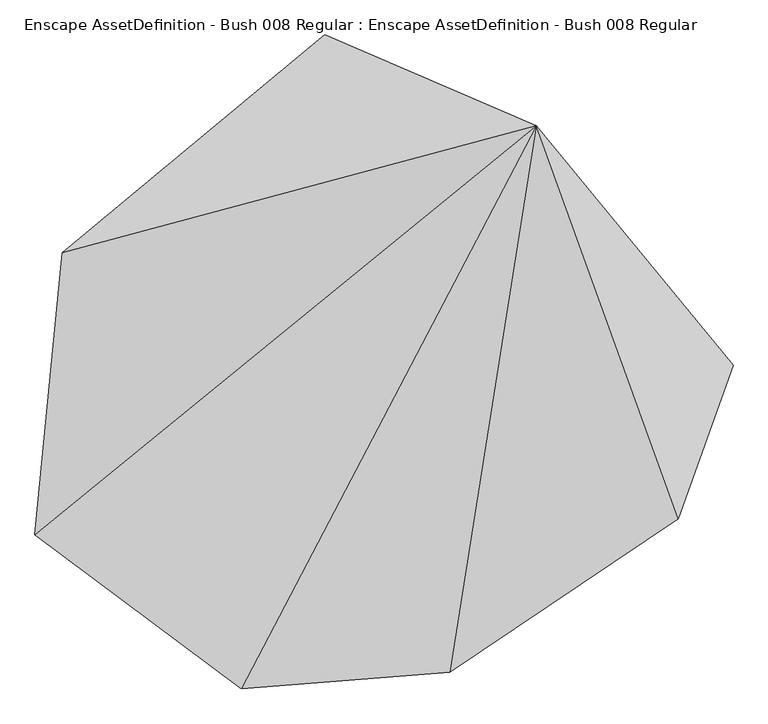
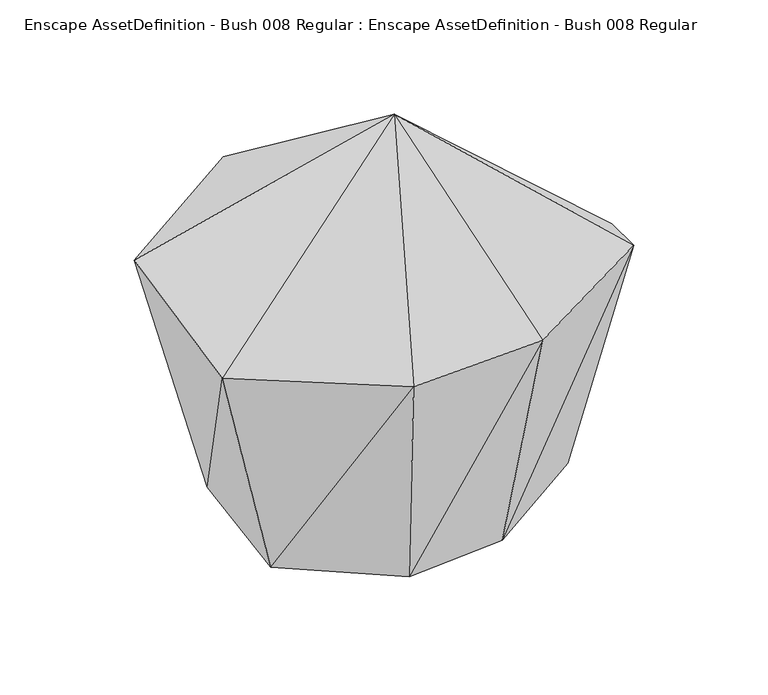
"""IFC4 building model written with IfcOpenShell, lengths in millimetres: geographic element geometry, Enscape AssetDefinition - Bush 008 Regular : Enscape AssetDefinition - Bush 008 Regular."""

from ifc_helpers import new_model, si_unit, origin, place, context, project, spatial, faceted_brep, source, transform, mapped, element, save


def enscape_assetdefinition_bush_008_regular_enscape_4d63b102(model_context):
    return source(origin(), model_context, "Body", "Brep", [
        faceted_brep([(-732.7302098, -362.3848855, 766.569972), (-488.0544245, 143.9245045, 0.0), (-529.4855833, -283.1877768, 0.0), (-675.306201, 229.6019644, 791.0672426), (-90.5457214, 473.4426737, 0.0), (229.8599929, 336.0404968, 0.0), (-300.0746369, -686.321795, 781.7997932), (-217.3293233, -516.9049501, 0.0), (319.7386861, 495.8788455, 779.6196342), (-124.3504807, 686.321795, 674.3021011), (527.8295279, -26.7513935, 0.0), (732.7302098, -6.9583626, 565.536499), (617.8262234, -329.4171691, 728.3439636), (138.3782178, -650.9299278, 766.2059665), (99.0101621, -491.3705885, 0.0), (444.9271858, -259.40153, 0.0)], [[[0, 1, 2]], [[3, 4, 1]], [[4, 5, 1]], [[1, 0, 3]], [[1, 5, 2]], [[6, 2, 7]], [[2, 6, 0]], [[2, 5, 7]], [[0, 8, 3]], [[8, 0, 6]], [[3, 8, 9]], [[4, 3, 9]], [[9, 5, 4]], [[5, 9, 8]], [[8, 10, 5]], [[11, 8, 12]], [[13, 8, 6]], [[8, 13, 12]], [[10, 8, 11]], [[7, 13, 6]], [[13, 7, 14]], [[7, 5, 14]], [[14, 12, 13]], [[12, 14, 15]], [[15, 11, 12]], [[11, 15, 10]], [[15, 5, 10]], [[14, 5, 15]]]),
    ])


if __name__ == "__main__":
    model = new_model("IFC4")
    model_context = context("Model", 3, world=origin())
    ifc_project = project(units=[si_unit("LENGTHUNIT", "METRE", prefix="MILLI")], contexts=[model_context])
    site = spatial("IfcSite", under=ifc_project)
    building = spatial("IfcBuilding", under=site)
    placement = place(None, origin())
    enscape_assetdefinition_bush_008_regular_enscape_shape = enscape_assetdefinition_bush_008_regular_enscape_4d63b102(model_context)
    element("IfcGeographicElement", 1, ObjectType="Enscape AssetDefinition - Bush 008 Regular : Enscape AssetDefinition - Bush 008 Regular", at=placement, inside=building, context=model_context, shape_type="MappedRepresentation", body=[
        mapped(enscape_assetdefinition_bush_008_regular_enscape_shape, transform((0.0, 0.0, 0.0), x_axis=(1.0, 0.0, 0.0), y_axis=(0.0, 1.0, 0.0), z_axis=(0.0, 0.0, 1.0))),
    ])
    save(model, "model.ifc")

# Revit data of these elements
# Type "Enscape AssetDefinition - Bush 008 Regular : Enscape AssetDefinition - Bush 008 Regular"
#   EnscapeAssetSource = "REMOTE"
#   EnscapeAssetId = "e105e822-0401-445c-9002-d8e0982bb1df"
#   Height = 0.791067 m
#   EnscapeNativeAssetHeight = 0.791067 m
#   Default Elevation = 0
